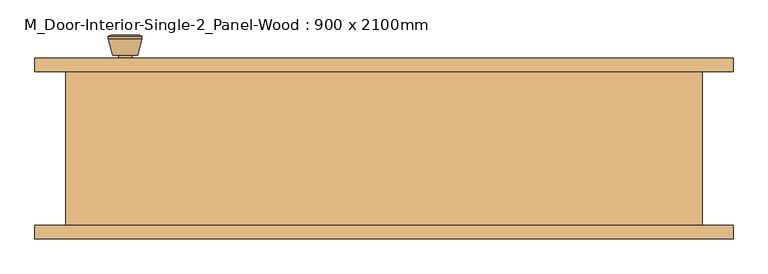
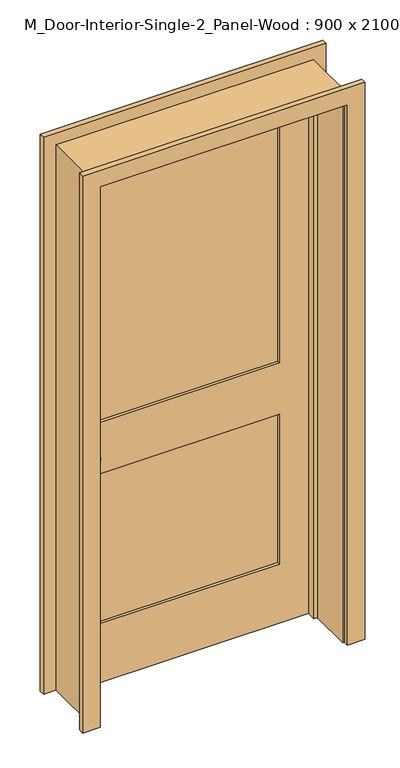
"""IFC4 building model written with IfcOpenShell, lengths in millimetres: door geometry, M_Door-Interior-Single-2_Panel-Wood : 900 x 2100mm."""

from ifc_helpers import new_model, si_unit, point, frame, frame_2d, origin, place, context, project, spatial, polyline, circle_curve, trimmed, segment, composite_curve, outline, extrude, faceted_brep, source, transform, mapped, element, save
from ifc_brep_helpers import plane_surface, cylinder_surface, revolved_surface, advanced_brep


def m_door_interior_single_2_panel_wood_900_x_2100mm_531a9286(model_context):
    return source(origin(), model_context, "Body", "SolidModel", [
        advanced_brep(
        [(-386.5, 70.825, 914.4), (-376.5, 70.825, 914.4), (-396.5, 70.825, 914.4), (-366.0241324, 21.825, 914.4), (-386.5, 21.825, 914.4), (-406.9758676, 21.825, 914.4), (-361.5, 23.6528681, 914.4), (-411.5, 23.6528681, 914.4), (-361.5, 27.1165463, 914.4), (-411.5, 27.1165463, 914.4), (-367.863764, 51.825, 914.4), (-405.136236, 51.825, 914.4), (-376.5, 51.825, 914.4), (-396.5, 51.825, 914.4)],
        [
            (0, 1),
            (1, 2, circle_curve(frame((-386.5, 70.825, 914.4), z_axis=(0.0, 1.0, 0.0), x_axis=(-1.0, 0.0, 0.0)), 10.0)),
            (2, 0),
            (2, 1, circle_curve(frame((-386.5, 70.825, 914.4), z_axis=(0.0, 1.0, 0.0), x_axis=(-1.0, 0.0, 0.0)), 10.0)),
            (3, 4),
            (4, 5),
            (5, 3, circle_curve(frame((-386.5, 21.825, 914.4), z_axis=(0.0, -1.0, 0.0), x_axis=(-1.0, 0.0, 0.0)), 20.4758676)),
            (3, 5, circle_curve(frame((-386.5, 21.825, 914.4), z_axis=(0.0, -1.0, 0.0), x_axis=(-1.0, 0.0, 0.0)), 20.4758676)),
            (6, 3),
            (5, 7),
            (7, 6, circle_curve(frame((-386.5, 23.6528681, 914.4), z_axis=(0.0, -1.0, 0.0), x_axis=(-1.0, 0.0, 0.0)), 25.0)),
            (6, 7, circle_curve(frame((-386.5, 23.6528681, 914.4), z_axis=(0.0, -1.0, 0.0), x_axis=(-1.0, 0.0, 0.0)), 25.0)),
            (8, 6),
            (7, 9),
            (9, 8, circle_curve(frame((-386.5, 27.1165463, 914.4), z_axis=(0.0, -1.0, 0.0), x_axis=(-1.0, 0.0, 0.0)), 25.0)),
            (8, 9, circle_curve(frame((-386.5, 27.1165463, 914.4), z_axis=(0.0, -1.0, 0.0), x_axis=(-1.0, 0.0, 0.0)), 25.0)),
            (10, 8),
            (9, 11),
            (11, 10, circle_curve(frame((-386.5, 51.825, 914.4), z_axis=(0.0, -1.0, 0.0), x_axis=(-1.0, 0.0, 0.0)), 18.636236)),
            (10, 11, circle_curve(frame((-386.5, 51.825, 914.4), z_axis=(0.0, -1.0, 0.0), x_axis=(-1.0, 0.0, 0.0)), 18.636236)),
            (12, 10),
            (11, 13),
            (13, 12, circle_curve(frame((-386.5, 51.825, 914.4), z_axis=(0.0, -1.0, 0.0), x_axis=(-1.0, 0.0, 0.0)), 10.0)),
            (12, 13, circle_curve(frame((-386.5, 51.825, 914.4), z_axis=(0.0, -1.0, 0.0), x_axis=(-1.0, 0.0, 0.0)), 10.0)),
            (1, 12),
            (13, 2),
        ],
        [
            plane_surface(frame((-386.5, 70.825, 914.4), z_axis=(0.0, 1.0, 0.0), x_axis=(-1.0, 0.0, 0.0))),
            plane_surface(frame((-386.5, 21.825, 914.4), z_axis=(0.0, -1.0, 0.0), x_axis=(-1.0, 0.0, 0.0))),
            revolved_surface(polyline([(-406.9758676, 21.825, 914.4), (-411.5, 23.6528681, 914.4)]), (-386.5, 70.825, 914.4), (0.0, 1.0, 0.0)),
            cylinder_surface(frame((-386.5, 70.825, 914.4), z_axis=(0.0, 1.0, 0.0), x_axis=(-1.0, 0.0, 0.0)), 25.0),
            revolved_surface(polyline([(-411.5, 27.1165463, 914.4), (-405.136236, 51.825, 914.4)]), (-386.5, 70.825, 914.4), (0.0, 1.0, 0.0)),
            plane_surface(frame((-386.5, 51.825, 914.4), z_axis=(0.0, 1.0, 0.0), x_axis=(-1.0, 0.0, 0.0))),
            cylinder_surface(frame((-386.5, 70.825, 914.4), z_axis=(0.0, 1.0, 0.0), x_axis=(-1.0, 0.0, 0.0)), 10.0),
        ],
        [
            (0, [[1, 2, 3]]),
            (0, [[-3, 4, -1]]),
            (1, [[5, 6, 7]]),
            (1, [[-6, -5, 8]]),
            (2, [[9, -7, 10, 11]]),
            (2, [[-10, -8, -9, 12]]),
            (3, [[13, -11, 14, 15]]),
            (3, [[-14, -12, -13, 16]]),
            (4, [[17, -15, 18, 19]]),
            (4, [[-18, -16, -17, 20]]),
            (5, [[21, -19, 22, 23]]),
            (5, [[-22, -20, -21, 24]]),
            (6, [[25, -23, 26, -2]]),
            (6, [[-26, -24, -25, -4]]),
        ],
    ),
        extrude(outline(composite_curve([segment(trimmed(circle_curve(frame_2d((914.4, -386.5)), 30.0), [point((914.4, -416.5))], [point((914.4, -356.5))], False, "CARTESIAN"), True, "CONTINUOUS"), segment(trimmed(circle_curve(frame_2d((914.4, -386.5)), 30.0), [point((914.4, -356.5))], [point((914.4, -416.5))], False, "CARTESIAN"), True, "CONTINUOUS")], self_intersect=False)), frame((0.0, 70.825, 0.0), z_axis=(0.0, 1.0, 0.0), x_axis=(0.0, 0.0, 1.0)), (0.0, 0.0, 1.0), 6.0),
        advanced_brep(
        [(-386.5, 117.825, 914.4), (-396.5, 117.825, 914.4), (-376.5, 117.825, 914.4), (-366.0241324, 166.825, 914.4), (-406.9758676, 166.825, 914.4), (-386.5, 166.825, 914.4), (-361.5, 164.9971319, 914.4), (-411.5, 164.9971319, 914.4), (-361.5, 161.5334537, 914.4), (-411.5, 161.5334537, 914.4), (-367.863764, 136.825, 914.4), (-405.136236, 136.825, 914.4), (-376.5, 136.825, 914.4), (-396.5, 136.825, 914.4)],
        [
            (0, 1),
            (1, 2, circle_curve(frame((-386.5, 117.825, 914.4), z_axis=(0.0, -1.0, 0.0), x_axis=(-1.0, 0.0, 0.0)), 10.0)),
            (2, 0),
            (2, 1, circle_curve(frame((-386.5, 117.825, 914.4), z_axis=(0.0, -1.0, 0.0), x_axis=(-1.0, 0.0, 0.0)), 10.0)),
            (3, 4, circle_curve(frame((-386.5, 166.825, 914.4), z_axis=(0.0, 1.0, 0.0), x_axis=(-1.0, 0.0, 0.0)), 20.4758676)),
            (4, 5),
            (5, 3),
            (4, 3, circle_curve(frame((-386.5, 166.825, 914.4), z_axis=(0.0, 1.0, 0.0), x_axis=(-1.0, 0.0, 0.0)), 20.4758676)),
            (6, 7, circle_curve(frame((-386.5, 164.9971319, 914.4), z_axis=(0.0, 1.0, 0.0), x_axis=(-1.0, 0.0, 0.0)), 25.0)),
            (7, 4),
            (3, 6),
            (7, 6, circle_curve(frame((-386.5, 164.9971319, 914.4), z_axis=(0.0, 1.0, 0.0), x_axis=(-1.0, 0.0, 0.0)), 25.0)),
            (8, 9, circle_curve(frame((-386.5, 161.5334537, 914.4), z_axis=(0.0, 1.0, 0.0), x_axis=(-1.0, 0.0, 0.0)), 25.0)),
            (9, 7),
            (6, 8),
            (9, 8, circle_curve(frame((-386.5, 161.5334537, 914.4), z_axis=(0.0, 1.0, 0.0), x_axis=(-1.0, 0.0, 0.0)), 25.0)),
            (10, 11, circle_curve(frame((-386.5, 136.825, 914.4), z_axis=(0.0, 1.0, 0.0), x_axis=(-1.0, 0.0, 0.0)), 18.636236)),
            (11, 9),
            (8, 10),
            (11, 10, circle_curve(frame((-386.5, 136.825, 914.4), z_axis=(0.0, 1.0, 0.0), x_axis=(-1.0, 0.0, 0.0)), 18.636236)),
            (12, 13, circle_curve(frame((-386.5, 136.825, 914.4), z_axis=(0.0, 1.0, 0.0), x_axis=(-1.0, 0.0, 0.0)), 10.0)),
            (13, 11),
            (10, 12),
            (13, 12, circle_curve(frame((-386.5, 136.825, 914.4), z_axis=(0.0, 1.0, 0.0), x_axis=(-1.0, 0.0, 0.0)), 10.0)),
            (1, 13),
            (12, 2),
        ],
        [
            plane_surface(frame((-386.5, 117.825, 914.4), z_axis=(0.0, -1.0, 0.0), x_axis=(-1.0, 0.0, 0.0))),
            plane_surface(frame((-386.5, 166.825, 914.4), z_axis=(0.0, 1.0, 0.0), x_axis=(-1.0, 0.0, 0.0))),
            revolved_surface(polyline([(-406.9758676, 166.825, 914.4), (-411.5, 164.9971319, 914.4)]), (-386.5, 117.825, 914.4), (0.0, -1.0, 0.0)),
            cylinder_surface(frame((-386.5, 117.825, 914.4), z_axis=(0.0, -1.0, 0.0), x_axis=(-1.0, 0.0, 0.0)), 25.0),
            revolved_surface(polyline([(-411.5, 161.5334537, 914.4), (-405.136236, 136.825, 914.4)]), (-386.5, 117.825, 914.4), (0.0, -1.0, 0.0)),
            plane_surface(frame((-386.5, 136.825, 914.4), z_axis=(0.0, -1.0, 0.0), x_axis=(-1.0, 0.0, 0.0))),
            cylinder_surface(frame((-386.5, 117.825, 914.4), z_axis=(0.0, -1.0, 0.0), x_axis=(-1.0, 0.0, 0.0)), 10.0),
        ],
        [
            (0, [[1, 2, 3]]),
            (0, [[-3, 4, -1]]),
            (1, [[5, 6, 7]]),
            (1, [[8, -7, -6]]),
            (2, [[9, 10, -5, 11]]),
            (2, [[12, -11, -8, -10]]),
            (3, [[13, 14, -9, 15]]),
            (3, [[16, -15, -12, -14]]),
            (4, [[17, 18, -13, 19]]),
            (4, [[20, -19, -16, -18]]),
            (5, [[21, 22, -17, 23]]),
            (5, [[24, -23, -20, -22]]),
            (6, [[-2, 25, -21, 26]]),
            (6, [[-4, -26, -24, -25]]),
        ],
    ),
        extrude(outline(composite_curve([segment(trimmed(circle_curve(frame_2d((914.4, -386.5)), 30.0), [point((914.4, -416.5))], [point((914.4, -356.5))], False, "CARTESIAN"), True, "CONTINUOUS"), segment(trimmed(circle_curve(frame_2d((914.4, -386.5)), 30.0), [point((914.4, -356.5))], [point((914.4, -416.5))], False, "CARTESIAN"), True, "CONTINUOUS")], self_intersect=False)), frame((0.0, 111.825, 0.0), z_axis=(0.0, 1.0, 0.0), x_axis=(0.0, 0.0, 1.0)), (0.0, 0.0, 1.0), 6.0),
        extrude(outline(polyline([(330.0, 88.4916667), (-330.0, 88.4916667), (-330.0, 100.1583333), (330.0, 100.1583333), (330.0, 88.4916667)])), frame((0.0, 0.0, 1014.4), z_axis=(0.0, 0.0, 1.0), x_axis=(1.0, 0.0, 0.0)), (0.0, 0.0, 1.0), 965.6),
        extrude(outline(polyline([(330.0, 88.4916667), (-330.0, 88.4916667), (-330.0, 100.1583333), (330.0, 100.1583333), (330.0, 88.4916667)])), frame((0.0, 0.0, 230.0), z_axis=(0.0, 0.0, 1.0), x_axis=(1.0, 0.0, 0.0)), (0.0, 0.0, 1.0), 584.4),
        extrude(outline(polyline([(2100.0, -450.0), (0.0, -450.0), (0.0, 450.0), (2100.0, 450.0), (2100.0, -450.0)]), holes=[polyline([(1980.0, -330.0), (1980.0, 330.0), (1014.4, 330.0), (1014.4, -330.0), (1980.0, -330.0)]), polyline([(814.4, -330.0), (814.4, 330.0), (230.0, 330.0), (230.0, -330.0), (814.4, -330.0)])]), frame((0.0, 76.825, 0.0), z_axis=(0.0, 1.0, 0.0), x_axis=(0.0, 0.0, 1.0)), (0.0, 0.0, 1.0), 35.0),
        faceted_brep([(475.0, 111.825, 0.0), (475.0, -118.175, 0.0), (450.0, -118.175, 0.0), (450.0, 41.9, 0.0), (437.3, 41.9, 0.0), (437.3, 76.825, 0.0), (450.0, 76.825, 0.0), (450.0, 111.825, 0.0), (475.0, 111.825, 2125.0), (475.0, -118.175, 2125.0), (-475.0, -118.175, 2125.0), (-475.0, -118.175, 0.0), (-450.0, -118.175, 0.0), (-450.0, -118.175, 2100.0), (450.0, -118.175, 2100.0), (450.0, 41.9, 2100.0), (-450.0, 41.9, 2100.0), (-450.0, 41.9, 0.0), (-437.3, 41.9, 0.0), (-437.3, 41.9, 2087.3), (437.3, 41.9, 2087.3), (437.3, 76.825, 2087.3), (-437.3, 76.825, 2087.3), (-437.3, 76.825, 0.0), (-450.0, 76.825, 0.0), (-450.0, 76.825, 2100.0), (450.0, 76.825, 2100.0), (450.0, 111.825, 2100.0), (-450.0, 111.825, 2100.0), (-450.0, 111.825, 0.0), (-475.0, 111.825, 0.0), (-475.0, 111.825, 2125.0)], [[[0, 1, 2, 3, 4, 5, 6, 7]], [[1, 0, 8, 9]], [[2, 1, 9, 10, 11, 12, 13, 14]], [[3, 2, 14, 15]], [[4, 3, 15, 16, 17, 18, 19, 20]], [[5, 4, 20, 21]], [[6, 5, 21, 22, 23, 24, 25, 26]], [[7, 6, 26, 27]], [[0, 7, 27, 28, 29, 30, 31, 8]], [[9, 8, 31, 10]], [[15, 14, 13, 16]], [[21, 20, 19, 22]], [[27, 26, 25, 28]], [[30, 29, 24, 23, 18, 17, 12, 11]], [[10, 31, 30, 11]], [[16, 13, 12, 17]], [[22, 19, 18, 23]], [[28, 25, 24, 29]]]),
        extrude(outline(polyline([(0.0, 456.35), (0.0, 521.35), (2171.35, 521.35), (2171.35, -521.35), (0.0, -521.35), (0.0, -456.35), (2106.35, -456.35), (2106.35, 456.35), (0.0, 456.35)])), frame((0.0, -138.175, 0.0), z_axis=(0.0, 1.0, 0.0), x_axis=(0.0, 0.0, 1.0)), (0.0, 0.0, 1.0), 20.0),
        extrude(outline(polyline([(0.0, 456.35), (0.0, 521.35), (2171.35, 521.35), (2171.35, -521.35), (0.0, -521.35), (0.0, -456.35), (2106.35, -456.35), (2106.35, 456.35), (0.0, 456.35)])), frame((0.0, 111.825, 0.0), z_axis=(0.0, 1.0, 0.0), x_axis=(0.0, 0.0, 1.0)), (0.0, 0.0, 1.0), 20.0),
    ])


if __name__ == "__main__":
    model = new_model("IFC4")
    model_context = context("Model", 3, world=origin())
    ifc_project = project(units=[si_unit("LENGTHUNIT", "METRE", prefix="MILLI")], contexts=[model_context])
    site = spatial("IfcSite", under=ifc_project)
    building = spatial("IfcBuilding", under=site)
    placement = place(None, origin())
    m_door_interior_single_2_panel_wood_900_x_2100mm_shape = m_door_interior_single_2_panel_wood_900_x_2100mm_531a9286(model_context)
    element("IfcDoor", 1, ObjectType="M_Door-Interior-Single-2_Panel-Wood : 900 x 2100mm", at=placement, inside=building, context=model_context, shape_type="MappedRepresentation", body=[
        mapped(m_door_interior_single_2_panel_wood_900_x_2100mm_shape, transform((0.0, 0.0, 0.0), x_axis=(1.0, 0.0, 0.0), y_axis=(0.0, 1.0, 0.0), z_axis=(0.0, 0.0, 1.0))),
    ])
    save(model, "model.ifc")

# Revit data of these elements
# Type "M_Door-Interior-Single-2_Panel-Wood : 900 x 2100mm"
#   Type Mark = "42"
#   Assembly Code = "C1020300"
#   Analytic Construction = "Wooden"
#   Top Rail = 12 cm
#   Thickness = 3.5 cm
#   Thermal Resistance (R) = 0.455703 (m²·K)/W
#   Swing Angle [instance default] = 90.00°
#   Stiles = 12 cm
#   Rough Width = 95 cm
#   Rough Height = 212.5 cm
#   Lock Rail = 20 cm
#   Height = 210 cm
#   Width = 90 cm
#   Heat Transfer Coefficient (U) = 2.19465 W/(m²·K)
#   Bottom Rail = 23 cm
#   Trim Material = Cherry
#   Panel Material = Cherry
#   Frame Material = Cherry
#   Door Handle Material = Aluminum
#   Visual Light Transmittance = 0
#   Solar Heat Gain Coefficient = 0
#   Wall Closure = (empty or 0)
#   Function = (empty or 0)
# Element 1 (IfcDoor, "M_Door-Interior-Single-2_Panel-Wood : 900 x 2100mm")
#   Materials on its faces: "Cherry", "Aluminum"
# Materials
#   "Cherry": class "Wood", colour RGB 226 177 128, transparency 0, Description = "Prunus Serotina", Cost = 0
#   "Aluminum": class "Metal", colour RGB 247 247 247, transparency 0, Description = "Aluminum 6061", Cost = 0
